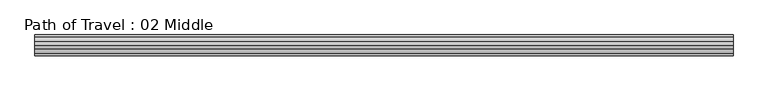
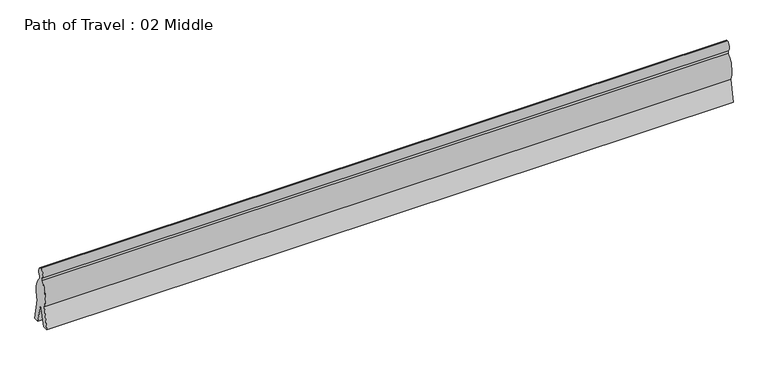
"""IFC4 building model written with IfcOpenShell, lengths in millimetres: proxy geometry, Path of Travel : 02 Middle."""

from ifc_helpers import new_model, si_unit, point, frame, origin, place, context, project, spatial, ellipse_curve, trimmed, source, transform, mapped, element, save
from ifc_brep_helpers import plane_surface, extruded_surface, advanced_brep


def path_of_travel_02_middle_47e593ae(model_context):
    return source(origin(), model_context, "Body", "AdvancedBrep", [
        advanced_brep(
        [(227.5554837, 0.0, 1727.2), (227.5554837, 42.9018657, 1436.6534209), (227.5554837, 42.9018657, 1363.4763406), (227.5554837, 184.1186263, 643.4144547), (227.5554837, 297.5699544, 0.0), (227.5554837, 145.6574193, 0.0), (227.5554837, 0.0, 584.2), (227.5554837, -145.6574193, 0.0), (227.5554837, -297.5699544, 0.0), (227.5554837, -184.1186263, 643.4144547), (227.5554837, -42.9018657, 1363.4763406), (227.5554837, -42.9018657, 1436.6534209), (20296.5311783, 0.0, 1727.2), (20296.5311783, -42.9018657, 1436.6534209), (20296.5311783, -42.9018657, 1363.4763406), (20296.5311783, -184.1186263, 643.4144547), (20296.5311783, -297.5699544, 0.0), (20296.5311783, -145.6574193, 0.0), (20296.5311783, 0.0, 584.2), (20296.5311783, 145.6574193, 0.0), (20296.5311783, 297.5699544, 0.0), (20296.5311783, 184.1186263, 643.4144547), (20296.5311783, 42.9018657, 1363.4763406), (20296.5311783, 42.9018657, 1436.6534209)],
        [
            (0, 1, ellipse_curve(frame((227.5554837, 0.0, 1574.8), z_axis=(-1.0, 0.0, 0.0), x_axis=(0.0, 0.0, 1.0)), 152.4, 101.6)),
            (1, 2),
            (2, 3, ellipse_curve(frame((227.5554837, 0.0, 914.4), z_axis=(-1.0, 0.0, 0.0), x_axis=(0.0, 0.0, -1.0)), 457.2, 228.6)),
            (3, 4),
            (4, 5),
            (5, 6),
            (6, 7),
            (7, 8),
            (8, 9),
            (9, 10, ellipse_curve(frame((227.5554837, 0.0, 914.4), z_axis=(-1.0, 0.0, 0.0), x_axis=(0.0, 0.0, -1.0)), 457.2, 228.6)),
            (10, 11),
            (11, 0, ellipse_curve(frame((227.5554837, 0.0, 1574.8), z_axis=(-1.0, 0.0, 0.0), x_axis=(0.0, 0.0, 1.0)), 152.4, 101.6)),
            (12, 13, ellipse_curve(frame((20296.5311783, 0.0, 1574.8), z_axis=(1.0, 0.0, 0.0), x_axis=(0.0, 0.0, 1.0)), 152.4, 101.6)),
            (13, 14),
            (14, 15, ellipse_curve(frame((20296.5311783, 0.0, 914.4), z_axis=(1.0, 0.0, 0.0), x_axis=(0.0, 0.0, -1.0)), 457.2, 228.6)),
            (15, 16),
            (16, 17),
            (17, 18),
            (18, 19),
            (19, 20),
            (20, 21),
            (21, 22, ellipse_curve(frame((20296.5311783, 0.0, 914.4), z_axis=(1.0, 0.0, 0.0), x_axis=(0.0, 0.0, -1.0)), 457.2, 228.6)),
            (22, 23),
            (23, 12, ellipse_curve(frame((20296.5311783, 0.0, 1574.8), z_axis=(1.0, 0.0, 0.0), x_axis=(0.0, 0.0, 1.0)), 152.4, 101.6)),
            (0, 12),
            (23, 1),
            (22, 2),
            (21, 3),
            (20, 4),
            (19, 5),
            (18, 6),
            (17, 7),
            (16, 8),
            (15, 9),
            (14, 10),
            (13, 11),
        ],
        [
            plane_surface(frame((227.5554837, 0.0, 0.0), z_axis=(-1.0, 0.0, 0.0), x_axis=(0.0, 0.0, 1.0))),
            plane_surface(frame((20296.5311783, 0.0, 0.0), z_axis=(1.0, 0.0, 0.0), x_axis=(0.0, 0.0, 1.0))),
            extruded_surface(trimmed(ellipse_curve(frame((20296.5311783, 0.0, 1574.8), z_axis=(-1.0, 0.0, 0.0), x_axis=(0.0, 0.0, 1.0)), 152.4, 101.6), [point((20296.5311783, 0.0, 1727.2))], [point((20296.5311783, 42.9018657, 1436.6534209))], True, "CARTESIAN"), (-20068.975694599998, 0.0, 0.0), 20068.975694599998),
            plane_surface(frame((227.5554837, 42.9018657, 1436.6534209), z_axis=(0.0, 1.0, 0.0), x_axis=(1.0, 0.0, 0.0))),
            extruded_surface(trimmed(ellipse_curve(frame((20296.5311783, 0.0, 914.4), z_axis=(-1.0, 0.0, 0.0), x_axis=(0.0, 0.0, -1.0)), 457.2, 228.6), [point((20296.5311783, 42.9018657, 1363.4763406))], [point((20296.5311783, 184.1186263, 643.4144547))], True, "CARTESIAN"), (-20068.975694599998, 0.0, 0.0), 20068.975694599998),
            plane_surface(frame((227.5554837, 184.1186263, 643.4144547), z_axis=(0.0, 0.9848077530122078, 0.17364817766693205), x_axis=(1.0, 0.0, 0.0))),
            plane_surface(frame((227.5554837, 297.5699544, 0.0), z_axis=(0.0, 0.0, -1.0), x_axis=(1.0, 0.0, 0.0))),
            plane_surface(frame((227.5554837, 145.6574193, 0.0), z_axis=(0.0, -0.9702957262760199, -0.2419218955995739), x_axis=(1.0, 0.0, 0.0))),
            plane_surface(frame((227.5554837, 0.0, 584.2), z_axis=(0.0, 0.9702957262759961, -0.24192189559966923), x_axis=(1.0, 0.0, 0.0))),
            plane_surface(frame((227.5554837, -145.6574193, 0.0), z_axis=(0.0, 0.0, -1.0), x_axis=(1.0, 0.0, 0.0))),
            plane_surface(frame((227.5554837, -297.5699544, 0.0), z_axis=(0.0, -0.984807753012208, 0.17364817766693066), x_axis=(1.0, 0.0, 0.0))),
            extruded_surface(trimmed(ellipse_curve(frame((20296.5311783, 0.0, 914.4), z_axis=(-1.0, 0.0, 0.0), x_axis=(0.0, 0.0, -1.0)), 457.2, 228.6), [point((20296.5311783, -184.1186263, 643.4144547))], [point((20296.5311783, -42.9018657, 1363.4763406))], True, "CARTESIAN"), (-20068.975694599998, 0.0, 0.0), 20068.975694599998),
            plane_surface(frame((227.5554837, -42.9018657, 1363.4763406), z_axis=(0.0, -1.0, 0.0), x_axis=(1.0, 0.0, 0.0))),
            extruded_surface(trimmed(ellipse_curve(frame((20296.5311783, 0.0, 1574.8), z_axis=(-1.0, 0.0, 0.0), x_axis=(0.0, 0.0, 1.0)), 152.4, 101.6), [point((20296.5311783, -42.9018657, 1436.6534209))], [point((20296.5311783, 0.0, 1727.2))], True, "CARTESIAN"), (-20068.975694599998, 0.0, 0.0), 20068.975694599998),
        ],
        [
            (0, [[1, 2, 3, 4, 5, 6, 7, 8, 9, 10, 11, 12]]),
            (1, [[13, 14, 15, 16, 17, 18, 19, 20, 21, 22, 23, 24]]),
            (2, [[-1, 25, -24, 26]]),
            (3, [[-2, -26, -23, 27]]),
            (4, [[-3, -27, -22, 28]]),
            (5, [[-4, -28, -21, 29]]),
            (6, [[-5, -29, -20, 30]]),
            (7, [[-6, -30, -19, 31]]),
            (8, [[-7, -31, -18, 32]]),
            (9, [[-8, -32, -17, 33]]),
            (10, [[-9, -33, -16, 34]]),
            (11, [[-10, -34, -15, 35]]),
            (12, [[-11, -35, -14, 36]]),
            (13, [[-12, -36, -13, -25]]),
        ],
    ),
    ])


if __name__ == "__main__":
    model = new_model("IFC4")
    model_context = context("Model", 3, world=origin())
    ifc_project = project(units=[si_unit("LENGTHUNIT", "METRE", prefix="MILLI")], contexts=[model_context])
    site = spatial("IfcSite", under=ifc_project)
    building = spatial("IfcBuilding", under=site)
    placement = place(None, origin())
    path_of_travel_02_middle_shape = path_of_travel_02_middle_47e593ae(model_context)
    element("IfcBuildingElementProxy", 1, Name="Path of Travel : 02 Middle", ObjectType="Path of Travel : 02 Middle", at=placement, inside=building, context=model_context, shape_type="MappedRepresentation", body=[
        mapped(path_of_travel_02_middle_shape, transform((0.0, 0.0, 0.0), x_axis=(1.0, 0.0, 0.0), y_axis=(0.0, 1.0, 0.0), z_axis=(0.0, 0.0, 1.0))),
    ])
    save(model, "model.ifc")

# Revit data of these elements
# Type "Path of Travel : 02 Middle"
#   Path of Egress [instance default] = 4' - 0"
#   built-in parameter 1001306 [instance default] = 4 (stored number, unit not read)
#   Dot at Start = no
#   Arrow in Middle = yes
#   Arrow at End = no
#   Egress Path = none
# Element 1 (IfcBuildingElementProxy, "Path of Travel : 02 Middle")
#   Path of Egress = 65' - 10.11715"
#   built-in parameter 1001306 = 65.8431 (stored number, unit not read)
#   Materials on its faces: "Egress Path Solid"
# Materials
#   "Egress Path Solid": class "Unassigned", colour RGB 255 128 64, transparency 0.75, Comments = "Rendering appearance not upgraded "
